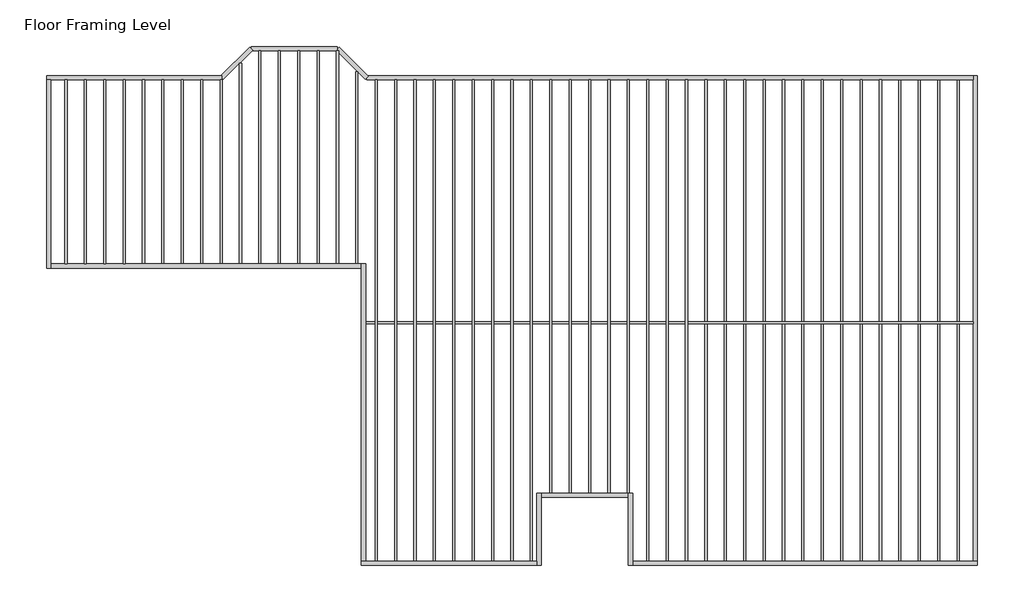
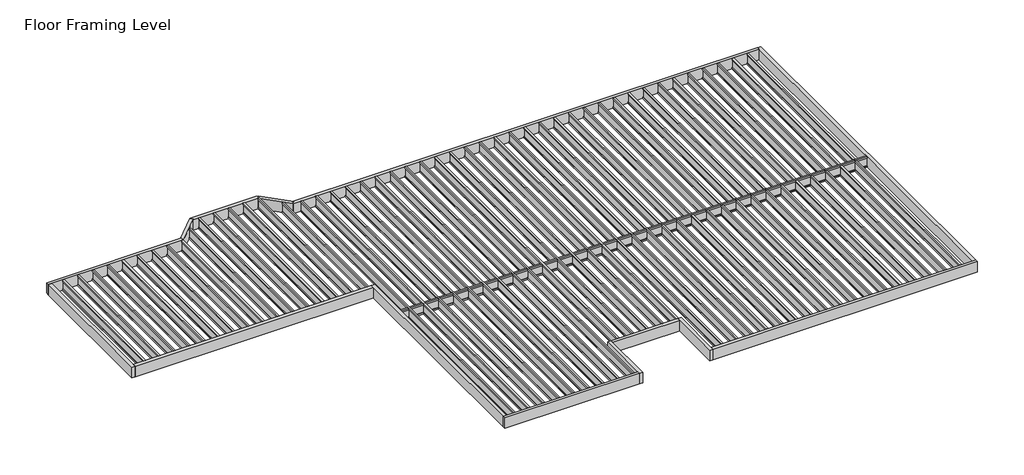
# One storey: 62 beams.
"""IFC4 building model written with IfcOpenShell, lengths in millimetres."""

import ifcopenshell
import ifcopenshell.guid

model = None  # the IFC model being written
_history = None  # IfcOwnerHistory: only IFC2X3 demands one
_inside = {}  # id of a spatial element -> (the spatial element, [elements in it])
_under = {}  # id of a project, library or spatial element -> (it, [spatial elements below it])
_declared = {}  # id of a project -> (the project, [libraries it declares])
_typed = {}  # id of a type object -> (the type object, [elements of that type])
_made_of = {}  # id of a material, layer set ... -> (it, [elements and type objects made of it])


def new_model(schema):
    """Start an empty IFC model of exactly this schema.

    Asked for "IFC4X3", IfcOpenShell would pick the latest addendum, in which some entities
    have other attributes; the version numbers below select the first issue.
    IFC2X3 requires an IfcOwnerHistory on every rooted entity: one is made here for all.
    """
    global model, _history
    if schema == "IFC4X3":
        model = ifcopenshell.file(schema_version=(4, 3, 0, 0))
    else:
        model = ifcopenshell.file(schema=schema)
    _inside.clear()
    _under.clear()
    _declared.clear()
    _typed.clear()
    _made_of.clear()
    _history = None
    if model.schema == "IFC2X3":
        org = make("IfcOrganization", Name="unknown")
        user = make(
            "IfcPersonAndOrganization",
            ThePerson=make("IfcPerson", FamilyName="unknown"),
            TheOrganization=org,
        )
        app = make(
            "IfcApplication",
            ApplicationDeveloper=org,
            Version="unknown",
            ApplicationFullName="unknown",
            ApplicationIdentifier="unknown",
        )
        _history = make(
            "IfcOwnerHistory",
            OwningUser=user,
            OwningApplication=app,
            ChangeAction="ADDED",
            CreationDate=0,
        )
    return model


def make(cls, **values):
    """One entity of the class cls with the attributes given. An attribute that is None is left unset."""
    return model.create_entity(
        cls, **{name: value for name, value in values.items() if value is not None}
    )


def rooted(cls, **values):
    """An entity with a GlobalId (a new one), such as an element, a storey or a relation."""
    return make(cls, GlobalId=ifcopenshell.guid.new(), OwnerHistory=_history, **values)


def si_unit(unit_type, name, prefix=None):
    """IfcSIUnit, for example si_unit("LENGTHUNIT", "METRE", prefix="MILLI")."""
    return make("IfcSIUnit", UnitType=unit_type, Prefix=prefix, Name=name)


def assignment(units):
    """IfcUnitAssignment: the units of a project."""
    return None if units is None else make("IfcUnitAssignment", Units=units)


def point(xyz):
    """IfcCartesianPoint."""
    return None if xyz is None else make("IfcCartesianPoint", Coordinates=xyz)


def direction(xyz):
    """IfcDirection."""
    return None if xyz is None else make("IfcDirection", DirectionRatios=xyz)


def frame(location, z_axis=None, x_axis=None):
    """IfcAxis2Placement3D, a coordinate frame: its origin and axes. An axis left out is left unset."""
    return make(
        "IfcAxis2Placement3D",
        Location=point(location),
        Axis=direction(z_axis),
        RefDirection=direction(x_axis),
    )


def origin():
    """The frame at (0, 0, 0) with its axes left unset."""
    return frame((0.0, 0.0, 0.0))


def place(relative_to, where):
    """IfcLocalPlacement: puts the frame where relative to a parent placement (None: the world)."""
    return make(
        "IfcLocalPlacement", PlacementRelTo=relative_to, RelativePlacement=where
    )


def context(
    kind, dimensions, precision=None, world=None, true_north=None, identifier=None
):
    """IfcGeometricRepresentationContext, for example the 3D "Model" context."""
    return make(
        "IfcGeometricRepresentationContext",
        ContextIdentifier=identifier,
        ContextType=kind,
        CoordinateSpaceDimension=dimensions,
        Precision=precision,
        WorldCoordinateSystem=world,
        TrueNorth=true_north,
    )


def project(units=None, contexts=None):
    """IfcProject with its units and contexts."""
    return rooted(
        "IfcProject",
        Name="project",
        RepresentationContexts=contexts,
        UnitsInContext=assignment(units),
    )


def spatial(cls, under=None, at=None, **own):
    """A site, building, storey or space (cls), placed at a placement, below another one or the project."""
    s = rooted(cls, ObjectPlacement=at, **own)
    if under is not None:
        _under.setdefault(under.id(), (under, []))[1].append(s)
    return s


def polyline(points):
    """IfcPolyline through the points."""
    return make("IfcPolyline", Points=[point(p) for p in points])


def outline(outer, holes=None, kind="AREA"):
    """IfcArbitraryClosedProfileDef: a profile drawn as a closed curve; with holes, ...WithVoids."""
    if holes is None:
        return make("IfcArbitraryClosedProfileDef", ProfileType=kind, OuterCurve=outer)
    return make(
        "IfcArbitraryProfileDefWithVoids",
        ProfileType=kind,
        OuterCurve=outer,
        InnerCurves=holes,
    )


def extrude(swept, where, along, depth):
    """IfcExtrudedAreaSolid: the profile swept, set in the frame where, extruded along a direction by depth."""
    return make(
        "IfcExtrudedAreaSolid",
        SweptArea=swept,
        Position=where,
        ExtrudedDirection=direction(along),
        Depth=depth,
    )


def shape(context_of_items, identifier, shape_type, items):
    """IfcShapeRepresentation: the items that make up one representation, for example the "Body"."""
    return make(
        "IfcShapeRepresentation",
        ContextOfItems=context_of_items,
        RepresentationIdentifier=identifier,
        RepresentationType=shape_type,
        Items=items,
    )


def source(mapping_origin, context_of_items, identifier, shape_type, items):
    """IfcRepresentationMap: a shape defined once, which mapped items show again and again."""
    return make(
        "IfcRepresentationMap",
        MappingOrigin=mapping_origin,
        MappedRepresentation=shape(context_of_items, identifier, shape_type, items),
    )


def transform(
    local_origin,
    x_axis=None,
    y_axis=None,
    z_axis=None,
    scale=None,
    scale2=None,
    scale3=None,
    uniform=True,
):
    """IfcCartesianTransformationOperator3D, or its non-uniform kind. x_axis, y_axis, z_axis: its Axis1, 2, 3."""
    if uniform:
        return make(
            "IfcCartesianTransformationOperator3D",
            Axis1=direction(x_axis),
            Axis2=direction(y_axis),
            LocalOrigin=point(local_origin),
            Scale=scale,
            Axis3=direction(z_axis),
        )
    return make(
        "IfcCartesianTransformationOperator3DnonUniform",
        Axis1=direction(x_axis),
        Axis2=direction(y_axis),
        LocalOrigin=point(local_origin),
        Scale=scale,
        Axis3=direction(z_axis),
        Scale2=scale2,
        Scale3=scale3,
    )


def mapped(mapping_source, mapping_target):
    """IfcMappedItem: shows the shape of a source again, moved by a transform."""
    return make(
        "IfcMappedItem", MappingSource=mapping_source, MappingTarget=mapping_target
    )


def made_of(thing, what):
    """Note that an element or type object is made of a material, layer set ...; save() writes the relation."""
    if what is not None:
        _made_of.setdefault(what.id(), (what, []))[1].append(thing)
    return thing


def element(
    cls,
    number,
    at=None,
    inside=None,
    cuts=None,
    type_object=None,
    material=None,
    context=None,
    identifier="Body",
    shape_type=None,
    held_by="IfcProductDefinitionShape",
    body=None,
    shapes=None,
    **own,
):
    """One element of the class cls, such as IfcWall. Its Tag is "e" and its number.

    at: its placement. inside: the storey or other place that contains it. cuts: it is an
    opening in that element (IfcRelVoidsElement). A single representation is given by context,
    identifier, shape_type and body (its items); several are given by shapes. held_by: the class
    of the entity that holds the representations. save() writes the other relations.
    """
    e = rooted(cls, Tag="e%d" % number, ObjectPlacement=at, **own)
    if body is not None:
        shapes = [shape(context, identifier, shape_type, body)]
    if shapes is not None:
        e.Representation = make(held_by, Representations=shapes)
    if inside is not None:
        _inside.setdefault(inside.id(), (inside, []))[1].append(e)
    if cuts is not None:
        rooted(
            "IfcRelVoidsElement", RelatingBuildingElement=cuts, RelatedOpeningElement=e
        )
    if type_object is not None:
        _typed.setdefault(type_object.id(), (type_object, []))[1].append(e)
    return made_of(e, material)


def aggregate(whole, parts):
    """IfcRelAggregates: a whole, such as a stair, and the parts it consists of."""
    return rooted("IfcRelAggregates", RelatingObject=whole, RelatedObjects=parts)


def save(model, path):
    """Write the relations noted so far, then the file.

    IfcRelAggregates (storeys below a building ...), IfcRelContainedInSpatialStructure (elements
    in a storey), IfcRelDefinesByType, IfcRelAssociatesMaterial and IfcRelDeclares: one each for
    every whole, place, type object, material and project.
    """
    for whole, parts in _under.values():
        aggregate(whole, parts)
    for where, things in _inside.values():
        rooted(
            "IfcRelContainedInSpatialStructure",
            RelatedElements=things,
            RelatingStructure=where,
        )
    for kind, things in _typed.values():
        rooted("IfcRelDefinesByType", RelatedObjects=things, RelatingType=kind)
    for what, things in _made_of.values():
        rooted("IfcRelAssociatesMaterial", RelatedObjects=things, RelatingMaterial=what)
    for by, libraries in _declared.values():
        rooted("IfcRelDeclares", RelatingContext=by, RelatedDefinitions=libraries)
    model.write(path)


def beam_585373de(model_context):
    return source(origin(), model_context, "Body", "SweptSolid", [
        extrude(outline(polyline([(755.65, 44.45), (755.65, -44.45), (-755.65, -44.45), (-755.65, 44.45), (755.65, 44.45)])), frame((0.0, 0.0, -150.8125), z_axis=(0.0, 0.0, 1.0), x_axis=(1.0, 0.0, 0.0)), (0.0, 0.0, 1.0), 301.625),
    ])


def beam_ce0f0212(model_context):
    return source(origin(), model_context, "Body", "SweptSolid", [
        extrude(outline(polyline([(5041.9, 44.45), (5041.9, -44.45), (-5130.8, -44.45), (-5130.8, 44.45), (5041.9, 44.45)])), frame((0.0, 0.0, -150.8125), z_axis=(0.0, 0.0, 1.0), x_axis=(1.0, 0.0, 0.0)), (0.0, 0.0, 1.0), 301.625),
    ])


def beam_45e17afb(model_context):
    return source(origin(), model_context, "Body", "SweptSolid", [
        extrude(outline(polyline([(3568.7, 44.45), (3568.7, -44.45), (-3657.6, -44.45), (-3657.6, 44.45), (3568.7, 44.45)])), frame((0.0, 0.0, -150.8125), z_axis=(0.0, 0.0, 1.0), x_axis=(1.0, 0.0, 0.0)), (0.0, 0.0, 1.0), 301.625),
    ])


def beam_b5369756(model_context):
    return source(origin(), model_context, "Body", "SweptSolid", [
        extrude(outline(polyline([(914.4, 44.45), (914.4, -44.45), (-914.4, -44.45), (-914.4, 44.45), (914.4, 44.45)])), frame((0.0, 0.0, -150.8125), z_axis=(0.0, 0.0, 1.0), x_axis=(1.0, 0.0, 0.0)), (0.0, 0.0, 1.0), 301.625),
    ])


def beam_28985cd7(model_context):
    return source(origin(), model_context, "Body", "SweptSolid", [
        extrude(outline(polyline([(1882.775, 44.45), (1882.775, -44.45), (-1793.875, -44.45), (-1793.875, 44.45), (1882.775, 44.45)])), frame((0.0, 0.0, -150.8125), z_axis=(0.0, 0.0, 1.0), x_axis=(1.0, 0.0, 0.0)), (0.0, 0.0, 1.0), 301.625),
    ])


def beam_51e41891(model_context):
    return source(origin(), model_context, "Body", "SweptSolid", [
        extrude(outline(polyline([(3159.125, 44.45), (3159.125, -44.45), (-3070.225, -44.45), (-3070.225, 44.45), (3159.125, 44.45)])), frame((0.0, 0.0, -150.8125), z_axis=(0.0, 0.0, 1.0), x_axis=(1.0, 0.0, 0.0)), (0.0, 0.0, 1.0), 301.625),
    ])


def beam_440427b1(model_context):
    return source(origin(), model_context, "Body", "SweptSolid", [
        extrude(outline(polyline([(3254.375, 44.45), (3254.375, -44.45), (-3254.375, -44.45), (-3254.375, 44.45), (3254.375, 44.45)])), frame((0.0, 0.0, -150.8125), z_axis=(0.0, 0.0, 1.0), x_axis=(1.0, 0.0, 0.0)), (0.0, 0.0, 1.0), 301.625),
    ])


def beam_dcf2d3fa(model_context):
    return source(origin(), model_context, "Body", "SweptSolid", [
        extrude(outline(polyline([(1927.225, 44.45), (1927.225, -44.45), (-2016.125, -44.45), (-2016.125, 44.45), (1927.225, 44.45)])), frame((0.0, 0.0, -150.8125), z_axis=(0.0, 0.0, 1.0), x_axis=(1.0, 0.0, 0.0)), (0.0, 0.0, 1.0), 301.625),
    ])


def beam_d6a2cfd4(model_context):
    return source(origin(), model_context, "Body", "SweptSolid", [
        extrude(outline(polyline([(431.0522938, 44.45), (431.0522938, -44.45), (-431.0522938, -44.45), (-431.0522938, 44.45), (431.0522938, 44.45)])), frame((0.0, 0.0, -150.8125), z_axis=(0.0, 0.0, 1.0), x_axis=(1.0, 0.0, 0.0)), (0.0, 0.0, 1.0), 301.625),
    ])


def beam_9835caef(model_context):
    return source(origin(), model_context, "Body", "SweptSolid", [
        extrude(outline(polyline([(1815.7808964, 44.45), (1815.7808964, -44.45), (-1860.2308964, -44.45), (-1860.2308964, 44.45), (1815.7808964, 44.45)])), frame((0.0, 0.0, -150.8125), z_axis=(0.0, 0.0, 1.0), x_axis=(1.0, 0.0, 0.0)), (0.0, 0.0, 1.0), 301.625),
    ])


def beam_6192414b(model_context):
    return source(origin(), model_context, "Body", "SweptSolid", [
        extrude(outline(polyline([(903.8789755, 44.45), (903.8789755, -44.45), (-906.5092316, -44.45), (-906.5092316, 44.45), (903.8789755, 44.45)])), frame((0.0, 0.0, -150.8125), z_axis=(0.0, 0.0, 1.0), x_axis=(1.0, 0.0, 0.0)), (0.0, 0.0, 1.0), 301.625),
    ])


def beam_06e53553(model_context):
    return source(origin(), model_context, "Body", "SweptSolid", [
        extrude(outline(polyline([(6332.8098719, 44.45), (6332.8098719, -44.45), (-6377.2598719, -44.45), (-6377.2598719, 44.45), (6332.8098719, 44.45)])), frame((0.0, 0.0, -150.8125), z_axis=(0.0, 0.0, 1.0), x_axis=(1.0, 0.0, 0.0)), (0.0, 0.0, 1.0), 301.625),
    ])


def plywood_web_joist_bldg_6241_1_3_4x11_7_8_b749f0c8(model_context):
    return source(origin(), model_context, "Body", "SweptSolid", [
        extrude(outline(polyline([(-22.225, 150.8125), (22.225, 150.8125), (22.225, 112.7125), (4.7625, 112.7125), (4.7625, 119.0625), (-4.7625, 119.0625), (-4.7625, 112.7125), (-22.225, 112.7125), (-22.225, 150.8125)])), frame((-5041.9, 0.0, 0.0), z_axis=(1.0, 0.0, 0.0), x_axis=(0.0, 1.0, 0.0)), (0.0, 0.0, 1.0), 10083.8),
        extrude(outline(polyline([(22.225, -112.7125), (22.225, -150.8125), (-22.225, -150.8125), (-22.225, -112.7125), (-4.7625, -112.7125), (-4.7625, -118.3285374), (4.7625, -118.3285374), (4.7625, -112.7125), (22.225, -112.7125)])), frame((-5041.9, 0.0, 0.0), z_axis=(1.0, 0.0, 0.0), x_axis=(0.0, 1.0, 0.0)), (0.0, 0.0, 1.0), 10083.8),
        extrude(outline(polyline([(5041.9, 4.7625), (5041.9, -4.7625), (-5041.9, -4.7625), (-5041.9, 4.7625), (5041.9, 4.7625)])), frame((0.0, 0.0, -118.3285374), z_axis=(0.0, 0.0, 1.0), x_axis=(1.0, 0.0, 0.0)), (0.0, 0.0, 1.0), 237.3910374),
    ])


def plywood_web_joist_bldg_6241_1_3_4x11_7_8_a6b37d20(model_context):
    return source(origin(), model_context, "Body", "SweptSolid", [
        extrude(outline(polyline([(-22.225, 150.8125), (22.225, 150.8125), (22.225, 112.7125), (4.7625, 112.7125), (4.7625, 119.0625), (-4.7625, 119.0625), (-4.7625, 112.7125), (-22.225, 112.7125), (-22.225, 150.8125)])), frame((-4330.7, 0.0, 0.0), z_axis=(1.0, 0.0, 0.0), x_axis=(0.0, 1.0, 0.0)), (0.0, 0.0, 1.0), 8661.4),
        extrude(outline(polyline([(22.225, -112.7125), (22.225, -150.8125), (-22.225, -150.8125), (-22.225, -112.7125), (-4.7625, -112.7125), (-4.7625, -118.3285374), (4.7625, -118.3285374), (4.7625, -112.7125), (22.225, -112.7125)])), frame((-4330.7, 0.0, 0.0), z_axis=(1.0, 0.0, 0.0), x_axis=(0.0, 1.0, 0.0)), (0.0, 0.0, 1.0), 8661.4),
        extrude(outline(polyline([(4330.7, 4.7625), (4330.7, -4.7625), (-4330.7, -4.7625), (-4330.7, 4.7625), (4330.7, 4.7625)])), frame((0.0, 0.0, -118.3285374), z_axis=(0.0, 0.0, 1.0), x_axis=(1.0, 0.0, 0.0)), (0.0, 0.0, 1.0), 237.3910374),
    ])


def plywood_web_joist_bldg_6241_1_3_4x11_7_8_9cf04d55(model_context):
    return source(origin(), model_context, "Body", "SweptSolid", [
        extrude(outline(polyline([(-22.225, 150.8125), (22.225, 150.8125), (22.225, 112.7125), (4.7625, 112.7125), (4.7625, 119.0625), (-4.7625, 119.0625), (-4.7625, 112.7125), (-22.225, 112.7125), (-22.225, 150.8125)])), frame((-1927.225, 0.0, 0.0), z_axis=(1.0, 0.0, 0.0), x_axis=(0.0, 1.0, 0.0)), (0.0, 0.0, 1.0), 3854.45),
        extrude(outline(polyline([(22.225, -112.7125), (22.225, -150.8125), (-22.225, -150.8125), (-22.225, -112.7125), (-4.7625, -112.7125), (-4.7625, -118.3285374), (4.7625, -118.3285374), (4.7625, -112.7125), (22.225, -112.7125)])), frame((-1927.225, 0.0, 0.0), z_axis=(1.0, 0.0, 0.0), x_axis=(0.0, 1.0, 0.0)), (0.0, 0.0, 1.0), 3854.45),
        extrude(outline(polyline([(1927.225, 4.7625), (1927.225, -4.7625), (-1927.225, -4.7625), (-1927.225, 4.7625), (1927.225, 4.7625)])), frame((0.0, 0.0, -118.3285374), z_axis=(0.0, 0.0, 1.0), x_axis=(1.0, 0.0, 0.0)), (0.0, 0.0, 1.0), 237.3910374),
    ])


def plywood_web_joist_bldg_6241_1_3_4x11_7_8_881987cb(model_context):
    return source(origin(), model_context, "Body", "SweptSolid", [
        extrude(outline(polyline([(-22.225, 150.8125), (22.225, 150.8125), (22.225, 112.7125), (4.7625, 112.7125), (4.7625, 119.0625), (-4.7625, 119.0625), (-4.7625, 112.7125), (-22.225, 112.7125), (-22.225, 150.8125)])), frame((-2121.2191036, 0.0, 0.0), z_axis=(1.0, 0.0, 0.0), x_axis=(0.0, 1.0, 0.0)), (0.0, 0.0, 1.0), 4201.8014143),
        extrude(outline(polyline([(22.225, -112.7125), (22.225, -150.8125), (-22.225, -150.8125), (-22.225, -112.7125), (-4.7625, -112.7125), (-4.7625, -118.3285374), (4.7625, -118.3285374), (4.7625, -112.7125), (22.225, -112.7125)])), frame((-2121.2191036, 0.0, 0.0), z_axis=(1.0, 0.0, 0.0), x_axis=(0.0, 1.0, 0.0)), (0.0, 0.0, 1.0), 4201.8014143),
        extrude(outline(polyline([(2080.5823107, 4.7625), (2080.5823107, -4.7625), (-2121.2191036, -4.7625), (-2121.2191036, 4.7625), (2080.5823107, 4.7625)])), frame((0.0, 0.0, -118.3285374), z_axis=(0.0, 0.0, 1.0), x_axis=(1.0, 0.0, 0.0)), (0.0, 0.0, 1.0), 237.3910374),
    ])


def plywood_web_joist_bldg_6241_1_3_4x11_7_8_a42695ab(model_context):
    return source(origin(), model_context, "Body", "SweptSolid", [
        extrude(outline(polyline([(-22.225, 150.8125), (22.225, 150.8125), (22.225, 112.7125), (4.7625, 112.7125), (4.7625, 119.0625), (-4.7625, 119.0625), (-4.7625, 112.7125), (-22.225, 112.7125), (-22.225, 150.8125)])), frame((-2232.025, 0.0, 0.0), z_axis=(1.0, 0.0, 0.0), x_axis=(0.0, 1.0, 0.0)), (0.0, 0.0, 1.0), 4464.05),
        extrude(outline(polyline([(22.225, -112.7125), (22.225, -150.8125), (-22.225, -150.8125), (-22.225, -112.7125), (-4.7625, -112.7125), (-4.7625, -118.3285374), (4.7625, -118.3285374), (4.7625, -112.7125), (22.225, -112.7125)])), frame((-2232.025, 0.0, 0.0), z_axis=(1.0, 0.0, 0.0), x_axis=(0.0, 1.0, 0.0)), (0.0, 0.0, 1.0), 4464.05),
        extrude(outline(polyline([(2232.025, 4.7625), (2232.025, -4.7625), (-2232.025, -4.7625), (-2232.025, 4.7625), (2232.025, 4.7625)])), frame((0.0, 0.0, -118.3285374), z_axis=(0.0, 0.0, 1.0), x_axis=(1.0, 0.0, 0.0)), (0.0, 0.0, 1.0), 237.3910374),
    ])


def plywood_web_joist_bldg_6241_1_3_4x11_7_8_0dc58311(model_context):
    return source(origin(), model_context, "Body", "SweptSolid", [
        extrude(outline(polyline([(-22.225, 150.8125), (22.225, 150.8125), (22.225, 112.7125), (4.7625, 112.7125), (4.7625, 119.0625), (-4.7625, 119.0625), (-4.7625, 112.7125), (-22.225, 112.7125), (-22.225, 150.8125)])), frame((-2030.1401281, 0.0, 0.0), z_axis=(1.0, 0.0, 0.0), x_axis=(0.0, 1.0, 0.0)), (0.0, 0.0, 1.0), 4019.6434633),
        extrude(outline(polyline([(22.225, -112.7125), (22.225, -150.8125), (-22.225, -150.8125), (-22.225, -112.7125), (-4.7625, -112.7125), (-4.7625, -118.3285374), (4.7625, -118.3285374), (4.7625, -112.7125), (22.225, -112.7125)])), frame((-2030.1401281, 0.0, 0.0), z_axis=(1.0, 0.0, 0.0), x_axis=(0.0, 1.0, 0.0)), (0.0, 0.0, 1.0), 4019.6434633),
        extrude(outline(polyline([(1989.5033352, 4.7625), (1989.5033352, -4.7625), (-2030.1401281, -4.7625), (-2030.1401281, 4.7625), (1989.5033352, 4.7625)])), frame((0.0, 0.0, -118.3285374), z_axis=(0.0, 0.0, 1.0), x_axis=(1.0, 0.0, 0.0)), (0.0, 0.0, 1.0), 237.3910374),
    ])


def plywood_web_joist_bldg_6241_1_3_4x11_7_8_0dbcbf17(model_context):
    return source(origin(), model_context, "Body", "SweptSolid", [
        extrude(outline(polyline([(-22.225, 150.8125), (22.225, 150.8125), (22.225, 112.7125), (4.7625, 112.7125), (4.7625, 119.0625), (-4.7625, 119.0625), (-4.7625, 112.7125), (-22.225, 112.7125), (-22.225, 150.8125)])), frame((-6365.875, 0.0, 0.0), z_axis=(1.0, 0.0, 0.0), x_axis=(0.0, 1.0, 0.0)), (0.0, 0.0, 1.0), 12731.75),
        extrude(outline(polyline([(22.225, -112.7125), (22.225, -150.8125), (-22.225, -150.8125), (-22.225, -112.7125), (-4.7625, -112.7125), (-4.7625, -118.3285374), (4.7625, -118.3285374), (4.7625, -112.7125), (22.225, -112.7125)])), frame((-6365.875, 0.0, 0.0), z_axis=(1.0, 0.0, 0.0), x_axis=(0.0, 1.0, 0.0)), (0.0, 0.0, 1.0), 12731.75),
        extrude(outline(polyline([(6365.875, 4.7625), (6365.875, -4.7625), (-6365.875, -4.7625), (-6365.875, 4.7625), (6365.875, 4.7625)])), frame((0.0, 0.0, -118.3285374), z_axis=(0.0, 0.0, 1.0), x_axis=(1.0, 0.0, 0.0)), (0.0, 0.0, 1.0), 237.3910374),
    ])


model = new_model("IFC4")

# Units and contexts
model_context = context("Model", 3, world=origin())
ifc_project = project(units=[si_unit("LENGTHUNIT", "METRE", prefix="MILLI")], contexts=[model_context])

# Site, building, storey
site = spatial("IfcSite", under=ifc_project)
building = spatial("IfcBuilding", under=site)
storey = spatial("IfcBuildingStorey", under=building, Name="Floor Framing Level", Elevation=-18.25625)

# Beams
placement = place(None, origin())
beam_shape = beam_585373de(model_context)
element("IfcBeam", 1, ObjectType="Dimension Lumber : BLDG 6241 Rim Board 11-7/8\"", at=placement, inside=storey, context=model_context, shape_type="MappedRepresentation", body=[
    mapped(beam_shape, transform((-5564.764829, -4298.2215886, -169.06875), x_axis=(0.0, 1.0, 0.0), y_axis=(-1.0, 0.0, 0.0), z_axis=(0.0, 0.0, 1.0))),
])
element("IfcBeam", 2, ObjectType="Dimension Lumber : BLDG 6241 Rim Board 11-7/8\"", at=placement, inside=storey, context=model_context, shape_type="MappedRepresentation", body=[
    mapped(beam_shape, transform((-7482.464829, -4298.2215886, -169.06875), x_axis=(0.0, -1.0, 0.0), y_axis=(1.0, 0.0, 0.0), z_axis=(0.0, 0.0, 1.0))),
])
beam_2_shape = beam_ce0f0212(model_context)
element("IfcBeam", 3, ObjectType="Dimension Lumber : BLDG 6241 Rim Board 11-7/8\"", at=placement, inside=storey, context=model_context, shape_type="MappedRepresentation", body=[
    mapped(beam_2_shape, transform((1661.535171, 76.9284114, -169.06875), x_axis=(0.0, -1.0, 0.0), y_axis=(1.0, 0.0, 0.0), z_axis=(0.0, 0.0, 1.0))),
])
beam_3_shape = beam_45e17afb(model_context)
element("IfcBeam", 4, ObjectType="Dimension Lumber : BLDG 6241 Rim Board 11-7/8\"", at=placement, inside=storey, context=model_context, shape_type="MappedRepresentation", body=[
    mapped(beam_3_shape, transform((-1951.614829, -5009.4215886, -169.06875), x_axis=(-1.0, 0.0, 0.0), y_axis=(0.0, -1.0, 0.0), z_axis=(0.0, 0.0, 1.0))),
])
beam_4_shape = beam_b5369756(model_context)
element("IfcBeam", 5, ObjectType="Dimension Lumber : BLDG 6241 Rim Board 11-7/8\"", at=placement, inside=storey, context=model_context, shape_type="MappedRepresentation", body=[
    mapped(beam_4_shape, transform((-6523.614829, -3587.0215886, -169.06875), x_axis=(-1.0, 0.0, 0.0), y_axis=(0.0, -1.0, 0.0), z_axis=(0.0, 0.0, 1.0))),
])
beam_5_shape = beam_28985cd7(model_context)
element("IfcBeam", 6, ObjectType="Dimension Lumber : BLDG 6241 Rim Board 11-7/8\"", at=placement, inside=storey, context=model_context, shape_type="MappedRepresentation", body=[
    mapped(beam_5_shape, transform((-9320.789829, -5009.4215886, -169.06875), x_axis=(-1.0, 0.0, 0.0), y_axis=(0.0, -1.0, 0.0), z_axis=(0.0, 0.0, 1.0))),
])
beam_6_shape = beam_51e41891(model_context)
element("IfcBeam", 7, ObjectType="Dimension Lumber : BLDG 6241 Rim Board 11-7/8\"", at=placement, inside=storey, context=model_context, shape_type="MappedRepresentation", body=[
    mapped(beam_6_shape, transform((-11159.114829, -1894.7465886, -169.06875), x_axis=(0.0, 1.0, 0.0), y_axis=(-1.0, 0.0, 0.0), z_axis=(0.0, 0.0, 1.0))),
])
beam_7_shape = beam_440427b1(model_context)
element("IfcBeam", 8, ObjectType="Dimension Lumber : BLDG 6241 Rim Board 11-7/8\"", at=placement, inside=storey, context=model_context, shape_type="MappedRepresentation", body=[
    mapped(beam_7_shape, transform((-14457.939829, 1219.9284114, -169.06875), x_axis=(-1.0, 0.0, 0.0), y_axis=(0.0, -1.0, 0.0), z_axis=(0.0, 0.0, 1.0))),
])
beam_8_shape = beam_dcf2d3fa(model_context)
element("IfcBeam", 9, ObjectType="Dimension Lumber : BLDG 6241 Rim Board 11-7/8\"", at=placement, inside=storey, context=model_context, shape_type="MappedRepresentation", body=[
    mapped(beam_8_shape, transform((-17756.764829, 3191.6034114, -169.06875), x_axis=(0.0, 1.0, 0.0), y_axis=(-1.0, 0.0, 0.0), z_axis=(0.0, 0.0, 1.0))),
])
beam_9_shape = beam_d6a2cfd4(model_context)
element("IfcBeam", 10, ObjectType="Dimension Lumber : BLDG 6241 Rim Board 11-7/8\"", at=placement, inside=storey, context=model_context, shape_type="MappedRepresentation", body=[
    mapped(beam_9_shape, transform((-13820.4030362, 5468.0784114, -169.06875), x_axis=(0.7071067811865488, 0.7071067811865464, 0.0), y_axis=(-0.7071067811865464, 0.7071067811865488, 0.0), z_axis=(0.0, 0.0, 1.0))),
])
element("IfcBeam", 11, ObjectType="Dimension Lumber : BLDG 6241 Rim Board 11-7/8\"", at=placement, inside=storey, context=model_context, shape_type="MappedRepresentation", body=[
    mapped(beam_9_shape, transform((-11397.7845729, 5468.0784114, -169.06875), x_axis=(0.7071067811865457, -0.7071067811865493, 0.0), y_axis=(0.7071067811865493, 0.7071067811865457, 0.0), z_axis=(0.0, 0.0, 1.0))),
])
beam_10_shape = beam_9835caef(model_context)
element("IfcBeam", 12, ObjectType="Dimension Lumber : BLDG 6241 Rim Board 11-7/8\"", at=placement, inside=storey, context=model_context, shape_type="MappedRepresentation", body=[
    mapped(beam_10_shape, transform((-15940.9839326, 5163.2784114, -169.06875), x_axis=(1.0, 0.0, 0.0), y_axis=(0.0, 1.0, 0.0), z_axis=(0.0, 0.0, 1.0))),
])
beam_11_shape = beam_6192414b(model_context)
element("IfcBeam", 13, ObjectType="Dimension Lumber : BLDG 6241 Rim Board 11-7/8\"", at=placement, inside=storey, context=model_context, shape_type="MappedRepresentation", body=[
    mapped(beam_11_shape, transform((-12609.0938046, 5772.8784114, -169.06875), x_axis=(1.0, 0.0, 0.0), y_axis=(0.0, 1.0, 0.0), z_axis=(0.0, 0.0, 1.0))),
])
beam_12_shape = beam_06e53553(model_context)
element("IfcBeam", 14, ObjectType="Dimension Lumber : BLDG 6241 Rim Board 11-7/8\"", at=placement, inside=storey, context=model_context, shape_type="MappedRepresentation", body=[
    mapped(beam_12_shape, transform((-4715.724701, 5163.2784114, -169.06875), x_axis=(1.0, 0.0, 0.0), y_axis=(0.0, 1.0, 0.0), z_axis=(0.0, 0.0, 1.0))),
])
plywood_web_joist_bldg_6241_1_3_4x11_7_8_shape = plywood_web_joist_bldg_6241_1_3_4x11_7_8_b749f0c8(model_context)
element("IfcBeam", 15, ObjectType="Plywood Web Joist : BLDG 6241 1 3/4x11 7/8", at=placement, inside=storey, context=model_context, shape_type="MappedRepresentation", body=[
    mapped(plywood_web_joist_bldg_6241_1_3_4x11_7_8_shape, transform((-10892.414829, 76.9284114, -169.06875), x_axis=(0.0, 1.0, 0.0), y_axis=(-1.0, 0.0, 0.0), z_axis=(0.0, 0.0, 1.0))),
])
element("IfcBeam", 16, ObjectType="Plywood Web Joist : BLDG 6241 1 3/4x11 7/8", at=placement, inside=storey, context=model_context, shape_type="MappedRepresentation", body=[
    mapped(plywood_web_joist_bldg_6241_1_3_4x11_7_8_shape, transform((-10486.014829, 76.9284114, -169.06875), x_axis=(0.0, 1.0, 0.0), y_axis=(-1.0, 0.0, 0.0), z_axis=(0.0, 0.0, 1.0))),
])
element("IfcBeam", 17, ObjectType="Plywood Web Joist : BLDG 6241 1 3/4x11 7/8", at=placement, inside=storey, context=model_context, shape_type="MappedRepresentation", body=[
    mapped(plywood_web_joist_bldg_6241_1_3_4x11_7_8_shape, transform((-10079.614829, 76.9284114, -169.06875), x_axis=(0.0, 1.0, 0.0), y_axis=(-1.0, 0.0, 0.0), z_axis=(0.0, 0.0, 1.0))),
])
element("IfcBeam", 18, ObjectType="Plywood Web Joist : BLDG 6241 1 3/4x11 7/8", at=placement, inside=storey, context=model_context, shape_type="MappedRepresentation", body=[
    mapped(plywood_web_joist_bldg_6241_1_3_4x11_7_8_shape, transform((-9673.214829, 76.9284114, -169.06875), x_axis=(0.0, 1.0, 0.0), y_axis=(-1.0, 0.0, 0.0), z_axis=(0.0, 0.0, 1.0))),
])
element("IfcBeam", 19, ObjectType="Plywood Web Joist : BLDG 6241 1 3/4x11 7/8", at=placement, inside=storey, context=model_context, shape_type="MappedRepresentation", body=[
    mapped(plywood_web_joist_bldg_6241_1_3_4x11_7_8_shape, transform((-9266.814829, 76.9284114, -169.06875), x_axis=(0.0, 1.0, 0.0), y_axis=(-1.0, 0.0, 0.0), z_axis=(0.0, 0.0, 1.0))),
])
element("IfcBeam", 20, ObjectType="Plywood Web Joist : BLDG 6241 1 3/4x11 7/8", at=placement, inside=storey, context=model_context, shape_type="MappedRepresentation", body=[
    mapped(plywood_web_joist_bldg_6241_1_3_4x11_7_8_shape, transform((-8860.414829, 76.9284114, -169.06875), x_axis=(0.0, 1.0, 0.0), y_axis=(-1.0, 0.0, 0.0), z_axis=(0.0, 0.0, 1.0))),
])
element("IfcBeam", 21, ObjectType="Plywood Web Joist : BLDG 6241 1 3/4x11 7/8", at=placement, inside=storey, context=model_context, shape_type="MappedRepresentation", body=[
    mapped(plywood_web_joist_bldg_6241_1_3_4x11_7_8_shape, transform((-8454.014829, 76.9284114, -169.06875), x_axis=(0.0, 1.0, 0.0), y_axis=(-1.0, 0.0, 0.0), z_axis=(0.0, 0.0, 1.0))),
])
element("IfcBeam", 22, ObjectType="Plywood Web Joist : BLDG 6241 1 3/4x11 7/8", at=placement, inside=storey, context=model_context, shape_type="MappedRepresentation", body=[
    mapped(plywood_web_joist_bldg_6241_1_3_4x11_7_8_shape, transform((-8047.614829, 76.9284114, -169.06875), x_axis=(0.0, 1.0, 0.0), y_axis=(-1.0, 0.0, 0.0), z_axis=(0.0, 0.0, 1.0))),
])
element("IfcBeam", 23, ObjectType="Plywood Web Joist : BLDG 6241 1 3/4x11 7/8", at=placement, inside=storey, context=model_context, shape_type="MappedRepresentation", body=[
    mapped(plywood_web_joist_bldg_6241_1_3_4x11_7_8_shape, transform((-7641.214829, 76.9284114, -169.06875), x_axis=(0.0, 1.0, 0.0), y_axis=(-1.0, 0.0, 0.0), z_axis=(0.0, 0.0, 1.0))),
])
element("IfcBeam", 24, ObjectType="Plywood Web Joist : BLDG 6241 1 3/4x11 7/8", at=placement, inside=storey, context=model_context, shape_type="MappedRepresentation", body=[
    mapped(plywood_web_joist_bldg_6241_1_3_4x11_7_8_shape, transform((-5202.814829, 76.9284114, -169.06875), x_axis=(0.0, 1.0, 0.0), y_axis=(-1.0, 0.0, 0.0), z_axis=(0.0, 0.0, 1.0))),
])
element("IfcBeam", 25, ObjectType="Plywood Web Joist : BLDG 6241 1 3/4x11 7/8", at=placement, inside=storey, context=model_context, shape_type="MappedRepresentation", body=[
    mapped(plywood_web_joist_bldg_6241_1_3_4x11_7_8_shape, transform((-4796.414829, 76.9284114, -169.06875), x_axis=(0.0, 1.0, 0.0), y_axis=(-1.0, 0.0, 0.0), z_axis=(0.0, 0.0, 1.0))),
])
element("IfcBeam", 26, ObjectType="Plywood Web Joist : BLDG 6241 1 3/4x11 7/8", at=placement, inside=storey, context=model_context, shape_type="MappedRepresentation", body=[
    mapped(plywood_web_joist_bldg_6241_1_3_4x11_7_8_shape, transform((-4390.014829, 76.9284114, -169.06875), x_axis=(0.0, 1.0, 0.0), y_axis=(-1.0, 0.0, 0.0), z_axis=(0.0, 0.0, 1.0))),
])
element("IfcBeam", 27, ObjectType="Plywood Web Joist : BLDG 6241 1 3/4x11 7/8", at=placement, inside=storey, context=model_context, shape_type="MappedRepresentation", body=[
    mapped(plywood_web_joist_bldg_6241_1_3_4x11_7_8_shape, transform((-3983.614829, 76.9284114, -169.06875), x_axis=(0.0, 1.0, 0.0), y_axis=(-1.0, 0.0, 0.0), z_axis=(0.0, 0.0, 1.0))),
])
element("IfcBeam", 28, ObjectType="Plywood Web Joist : BLDG 6241 1 3/4x11 7/8", at=placement, inside=storey, context=model_context, shape_type="MappedRepresentation", body=[
    mapped(plywood_web_joist_bldg_6241_1_3_4x11_7_8_shape, transform((-3577.214829, 76.9284114, -169.06875), x_axis=(0.0, 1.0, 0.0), y_axis=(-1.0, 0.0, 0.0), z_axis=(0.0, 0.0, 1.0))),
])
element("IfcBeam", 29, ObjectType="Plywood Web Joist : BLDG 6241 1 3/4x11 7/8", at=placement, inside=storey, context=model_context, shape_type="MappedRepresentation", body=[
    mapped(plywood_web_joist_bldg_6241_1_3_4x11_7_8_shape, transform((-3170.814829, 76.9284114, -169.06875), x_axis=(0.0, 1.0, 0.0), y_axis=(-1.0, 0.0, 0.0), z_axis=(0.0, 0.0, 1.0))),
])
element("IfcBeam", 30, ObjectType="Plywood Web Joist : BLDG 6241 1 3/4x11 7/8", at=placement, inside=storey, context=model_context, shape_type="MappedRepresentation", body=[
    mapped(plywood_web_joist_bldg_6241_1_3_4x11_7_8_shape, transform((-2764.414829, 76.9284114, -169.06875), x_axis=(0.0, 1.0, 0.0), y_axis=(-1.0, 0.0, 0.0), z_axis=(0.0, 0.0, 1.0))),
])
element("IfcBeam", 31, ObjectType="Plywood Web Joist : BLDG 6241 1 3/4x11 7/8", at=placement, inside=storey, context=model_context, shape_type="MappedRepresentation", body=[
    mapped(plywood_web_joist_bldg_6241_1_3_4x11_7_8_shape, transform((-2358.014829, 76.9284114, -169.06875), x_axis=(0.0, 1.0, 0.0), y_axis=(-1.0, 0.0, 0.0), z_axis=(0.0, 0.0, 1.0))),
])
element("IfcBeam", 32, ObjectType="Plywood Web Joist : BLDG 6241 1 3/4x11 7/8", at=placement, inside=storey, context=model_context, shape_type="MappedRepresentation", body=[
    mapped(plywood_web_joist_bldg_6241_1_3_4x11_7_8_shape, transform((-1951.614829, 76.9284114, -169.06875), x_axis=(0.0, 1.0, 0.0), y_axis=(-1.0, 0.0, 0.0), z_axis=(0.0, 0.0, 1.0))),
])
element("IfcBeam", 33, ObjectType="Plywood Web Joist : BLDG 6241 1 3/4x11 7/8", at=placement, inside=storey, context=model_context, shape_type="MappedRepresentation", body=[
    mapped(plywood_web_joist_bldg_6241_1_3_4x11_7_8_shape, transform((-1545.214829, 76.9284114, -169.06875), x_axis=(0.0, 1.0, 0.0), y_axis=(-1.0, 0.0, 0.0), z_axis=(0.0, 0.0, 1.0))),
])
element("IfcBeam", 34, ObjectType="Plywood Web Joist : BLDG 6241 1 3/4x11 7/8", at=placement, inside=storey, context=model_context, shape_type="MappedRepresentation", body=[
    mapped(plywood_web_joist_bldg_6241_1_3_4x11_7_8_shape, transform((-1138.814829, 76.9284114, -169.06875), x_axis=(0.0, 1.0, 0.0), y_axis=(-1.0, 0.0, 0.0), z_axis=(0.0, 0.0, 1.0))),
])
element("IfcBeam", 35, ObjectType="Plywood Web Joist : BLDG 6241 1 3/4x11 7/8", at=placement, inside=storey, context=model_context, shape_type="MappedRepresentation", body=[
    mapped(plywood_web_joist_bldg_6241_1_3_4x11_7_8_shape, transform((-732.414829, 76.9284114, -169.06875), x_axis=(0.0, 1.0, 0.0), y_axis=(-1.0, 0.0, 0.0), z_axis=(0.0, 0.0, 1.0))),
])
element("IfcBeam", 36, ObjectType="Plywood Web Joist : BLDG 6241 1 3/4x11 7/8", at=placement, inside=storey, context=model_context, shape_type="MappedRepresentation", body=[
    mapped(plywood_web_joist_bldg_6241_1_3_4x11_7_8_shape, transform((-326.014829, 76.9284114, -169.06875), x_axis=(0.0, 1.0, 0.0), y_axis=(-1.0, 0.0, 0.0), z_axis=(0.0, 0.0, 1.0))),
])
element("IfcBeam", 37, ObjectType="Plywood Web Joist : BLDG 6241 1 3/4x11 7/8", at=placement, inside=storey, context=model_context, shape_type="MappedRepresentation", body=[
    mapped(plywood_web_joist_bldg_6241_1_3_4x11_7_8_shape, transform((80.385171, 76.9284114, -169.06875), x_axis=(0.0, 1.0, 0.0), y_axis=(-1.0, 0.0, 0.0), z_axis=(0.0, 0.0, 1.0))),
])
element("IfcBeam", 38, ObjectType="Plywood Web Joist : BLDG 6241 1 3/4x11 7/8", at=placement, inside=storey, context=model_context, shape_type="MappedRepresentation", body=[
    mapped(plywood_web_joist_bldg_6241_1_3_4x11_7_8_shape, transform((486.785171, 76.9284114, -169.06875), x_axis=(0.0, 1.0, 0.0), y_axis=(-1.0, 0.0, 0.0), z_axis=(0.0, 0.0, 1.0))),
])
element("IfcBeam", 39, ObjectType="Plywood Web Joist : BLDG 6241 1 3/4x11 7/8", at=placement, inside=storey, context=model_context, shape_type="MappedRepresentation", body=[
    mapped(plywood_web_joist_bldg_6241_1_3_4x11_7_8_shape, transform((893.185171, 76.9284114, -169.06875), x_axis=(0.0, 1.0, 0.0), y_axis=(-1.0, 0.0, 0.0), z_axis=(0.0, 0.0, 1.0))),
])
element("IfcBeam", 40, ObjectType="Plywood Web Joist : BLDG 6241 1 3/4x11 7/8", at=placement, inside=storey, context=model_context, shape_type="MappedRepresentation", body=[
    mapped(plywood_web_joist_bldg_6241_1_3_4x11_7_8_shape, transform((1299.585171, 76.9284114, -169.06875), x_axis=(0.0, 1.0, 0.0), y_axis=(-1.0, 0.0, 0.0), z_axis=(0.0, 0.0, 1.0))),
])
plywood_web_joist_bldg_6241_1_3_4x11_7_8_2_shape = plywood_web_joist_bldg_6241_1_3_4x11_7_8_a6b37d20(model_context)
element("IfcBeam", 41, ObjectType="Plywood Web Joist : BLDG 6241 1 3/4x11 7/8", at=placement, inside=storey, context=model_context, shape_type="MappedRepresentation", body=[
    mapped(plywood_web_joist_bldg_6241_1_3_4x11_7_8_2_shape, transform((-7234.814829, 788.1284114, -169.06875), x_axis=(0.0, 1.0, 0.0), y_axis=(-1.0, 0.0, 0.0), z_axis=(0.0, 0.0, 1.0))),
])
element("IfcBeam", 42, ObjectType="Plywood Web Joist : BLDG 6241 1 3/4x11 7/8", at=placement, inside=storey, context=model_context, shape_type="MappedRepresentation", body=[
    mapped(plywood_web_joist_bldg_6241_1_3_4x11_7_8_2_shape, transform((-6828.414829, 788.1284114, -169.06875), x_axis=(0.0, 1.0, 0.0), y_axis=(-1.0, 0.0, 0.0), z_axis=(0.0, 0.0, 1.0))),
])
element("IfcBeam", 43, ObjectType="Plywood Web Joist : BLDG 6241 1 3/4x11 7/8", at=placement, inside=storey, context=model_context, shape_type="MappedRepresentation", body=[
    mapped(plywood_web_joist_bldg_6241_1_3_4x11_7_8_2_shape, transform((-6422.014829, 788.1284114, -169.06875), x_axis=(0.0, 1.0, 0.0), y_axis=(-1.0, 0.0, 0.0), z_axis=(0.0, 0.0, 1.0))),
])
element("IfcBeam", 44, ObjectType="Plywood Web Joist : BLDG 6241 1 3/4x11 7/8", at=placement, inside=storey, context=model_context, shape_type="MappedRepresentation", body=[
    mapped(plywood_web_joist_bldg_6241_1_3_4x11_7_8_2_shape, transform((-6015.614829, 788.1284114, -169.06875), x_axis=(0.0, 1.0, 0.0), y_axis=(-1.0, 0.0, 0.0), z_axis=(0.0, 0.0, 1.0))),
])
element("IfcBeam", 45, ObjectType="Plywood Web Joist : BLDG 6241 1 3/4x11 7/8", at=placement, inside=storey, context=model_context, shape_type="MappedRepresentation", body=[
    mapped(plywood_web_joist_bldg_6241_1_3_4x11_7_8_2_shape, transform((-5609.214829, 788.1284114, -169.06875), x_axis=(0.0, 1.0, 0.0), y_axis=(-1.0, 0.0, 0.0), z_axis=(0.0, 0.0, 1.0))),
])
plywood_web_joist_bldg_6241_1_3_4x11_7_8_3_shape = plywood_web_joist_bldg_6241_1_3_4x11_7_8_9cf04d55(model_context)
element("IfcBeam", 46, ObjectType="Plywood Web Joist : BLDG 6241 1 3/4x11 7/8", at=placement, inside=storey, context=model_context, shape_type="MappedRepresentation", body=[
    mapped(plywood_web_joist_bldg_6241_1_3_4x11_7_8_3_shape, transform((-17394.814829, 3191.6034114, -169.06875), x_axis=(0.0, 1.0, 0.0), y_axis=(-1.0, 0.0, 0.0), z_axis=(0.0, 0.0, 1.0))),
])
element("IfcBeam", 47, ObjectType="Plywood Web Joist : BLDG 6241 1 3/4x11 7/8", at=placement, inside=storey, context=model_context, shape_type="MappedRepresentation", body=[
    mapped(plywood_web_joist_bldg_6241_1_3_4x11_7_8_3_shape, transform((-16988.414829, 3191.6034114, -169.06875), x_axis=(0.0, 1.0, 0.0), y_axis=(-1.0, 0.0, 0.0), z_axis=(0.0, 0.0, 1.0))),
])
element("IfcBeam", 48, ObjectType="Plywood Web Joist : BLDG 6241 1 3/4x11 7/8", at=placement, inside=storey, context=model_context, shape_type="MappedRepresentation", body=[
    mapped(plywood_web_joist_bldg_6241_1_3_4x11_7_8_3_shape, transform((-16582.014829, 3191.6034114, -169.06875), x_axis=(0.0, 1.0, 0.0), y_axis=(-1.0, 0.0, 0.0), z_axis=(0.0, 0.0, 1.0))),
])
element("IfcBeam", 49, ObjectType="Plywood Web Joist : BLDG 6241 1 3/4x11 7/8", at=placement, inside=storey, context=model_context, shape_type="MappedRepresentation", body=[
    mapped(plywood_web_joist_bldg_6241_1_3_4x11_7_8_3_shape, transform((-16175.614829, 3191.6034114, -169.06875), x_axis=(0.0, 1.0, 0.0), y_axis=(-1.0, 0.0, 0.0), z_axis=(0.0, 0.0, 1.0))),
])
element("IfcBeam", 50, ObjectType="Plywood Web Joist : BLDG 6241 1 3/4x11 7/8", at=placement, inside=storey, context=model_context, shape_type="MappedRepresentation", body=[
    mapped(plywood_web_joist_bldg_6241_1_3_4x11_7_8_3_shape, transform((-15769.214829, 3191.6034114, -169.06875), x_axis=(0.0, 1.0, 0.0), y_axis=(-1.0, 0.0, 0.0), z_axis=(0.0, 0.0, 1.0))),
])
element("IfcBeam", 51, ObjectType="Plywood Web Joist : BLDG 6241 1 3/4x11 7/8", at=placement, inside=storey, context=model_context, shape_type="MappedRepresentation", body=[
    mapped(plywood_web_joist_bldg_6241_1_3_4x11_7_8_3_shape, transform((-15362.814829, 3191.6034114, -169.06875), x_axis=(0.0, 1.0, 0.0), y_axis=(-1.0, 0.0, 0.0), z_axis=(0.0, 0.0, 1.0))),
])
element("IfcBeam", 52, ObjectType="Plywood Web Joist : BLDG 6241 1 3/4x11 7/8", at=placement, inside=storey, context=model_context, shape_type="MappedRepresentation", body=[
    mapped(plywood_web_joist_bldg_6241_1_3_4x11_7_8_3_shape, transform((-14956.414829, 3191.6034114, -169.06875), x_axis=(0.0, 1.0, 0.0), y_axis=(-1.0, 0.0, 0.0), z_axis=(0.0, 0.0, 1.0))),
])
element("IfcBeam", 53, ObjectType="Plywood Web Joist : BLDG 6241 1 3/4x11 7/8", at=placement, inside=storey, context=model_context, shape_type="MappedRepresentation", body=[
    mapped(plywood_web_joist_bldg_6241_1_3_4x11_7_8_3_shape, transform((-14550.014829, 3191.6034114, -169.06875), x_axis=(0.0, 1.0, 0.0), y_axis=(-1.0, 0.0, 0.0), z_axis=(0.0, 0.0, 1.0))),
])
element("IfcBeam", 54, ObjectType="Plywood Web Joist : BLDG 6241 1 3/4x11 7/8", at=placement, inside=storey, context=model_context, shape_type="MappedRepresentation", body=[
    mapped(plywood_web_joist_bldg_6241_1_3_4x11_7_8_3_shape, transform((-14143.614829, 3191.6034114, -169.06875), x_axis=(0.0, 1.0, 0.0), y_axis=(-1.0, 0.0, 0.0), z_axis=(0.0, 0.0, 1.0))),
])
plywood_web_joist_bldg_6241_1_3_4x11_7_8_4_shape = plywood_web_joist_bldg_6241_1_3_4x11_7_8_881987cb(model_context)
element("IfcBeam", 55, ObjectType="Plywood Web Joist : BLDG 6241 1 3/4x11 7/8", at=placement, inside=storey, context=model_context, shape_type="MappedRepresentation", body=[
    mapped(plywood_web_joist_bldg_6241_1_3_4x11_7_8_4_shape, transform((-13737.214829, 3385.5975149, -169.06875), x_axis=(0.0, 1.0, 0.0), y_axis=(-1.0, 0.0, 0.0), z_axis=(0.0, 0.0, 1.0))),
])
plywood_web_joist_bldg_6241_1_3_4x11_7_8_5_shape = plywood_web_joist_bldg_6241_1_3_4x11_7_8_a42695ab(model_context)
element("IfcBeam", 56, ObjectType="Plywood Web Joist : BLDG 6241 1 3/4x11 7/8", at=placement, inside=storey, context=model_context, shape_type="MappedRepresentation", body=[
    mapped(plywood_web_joist_bldg_6241_1_3_4x11_7_8_5_shape, transform((-13330.814829, 3496.4034114, -169.06875), x_axis=(0.0, 1.0, 0.0), y_axis=(-1.0, 0.0, 0.0), z_axis=(0.0, 0.0, 1.0))),
])
element("IfcBeam", 57, ObjectType="Plywood Web Joist : BLDG 6241 1 3/4x11 7/8", at=placement, inside=storey, context=model_context, shape_type="MappedRepresentation", body=[
    mapped(plywood_web_joist_bldg_6241_1_3_4x11_7_8_5_shape, transform((-12924.414829, 3496.4034114, -169.06875), x_axis=(0.0, 1.0, 0.0), y_axis=(-1.0, 0.0, 0.0), z_axis=(0.0, 0.0, 1.0))),
])
element("IfcBeam", 58, ObjectType="Plywood Web Joist : BLDG 6241 1 3/4x11 7/8", at=placement, inside=storey, context=model_context, shape_type="MappedRepresentation", body=[
    mapped(plywood_web_joist_bldg_6241_1_3_4x11_7_8_5_shape, transform((-12518.014829, 3496.4034114, -169.06875), x_axis=(0.0, 1.0, 0.0), y_axis=(-1.0, 0.0, 0.0), z_axis=(0.0, 0.0, 1.0))),
])
element("IfcBeam", 59, ObjectType="Plywood Web Joist : BLDG 6241 1 3/4x11 7/8", at=placement, inside=storey, context=model_context, shape_type="MappedRepresentation", body=[
    mapped(plywood_web_joist_bldg_6241_1_3_4x11_7_8_5_shape, transform((-12111.614829, 3496.4034114, -169.06875), x_axis=(0.0, 1.0, 0.0), y_axis=(-1.0, 0.0, 0.0), z_axis=(0.0, 0.0, 1.0))),
])
element("IfcBeam", 60, ObjectType="Plywood Web Joist : BLDG 6241 1 3/4x11 7/8", at=placement, inside=storey, context=model_context, shape_type="MappedRepresentation", body=[
    mapped(plywood_web_joist_bldg_6241_1_3_4x11_7_8_5_shape, transform((-11705.214829, 3496.4034114, -169.06875), x_axis=(0.0, 1.0, 0.0), y_axis=(-1.0, 0.0, 0.0), z_axis=(0.0, 0.0, 1.0))),
])
plywood_web_joist_bldg_6241_1_3_4x11_7_8_6_shape = plywood_web_joist_bldg_6241_1_3_4x11_7_8_0dc58311(model_context)
element("IfcBeam", 61, ObjectType="Plywood Web Joist : BLDG 6241 1 3/4x11 7/8", at=placement, inside=storey, context=model_context, shape_type="MappedRepresentation", body=[
    mapped(plywood_web_joist_bldg_6241_1_3_4x11_7_8_6_shape, transform((-11298.814829, 3294.5185394, -169.06875), x_axis=(0.0, 1.0, 0.0), y_axis=(-1.0, 0.0, 0.0), z_axis=(0.0, 0.0, 1.0))),
])
plywood_web_joist_bldg_6241_1_3_4x11_7_8_7_shape = plywood_web_joist_bldg_6241_1_3_4x11_7_8_0dbcbf17(model_context)
element("IfcBeam", 62, ObjectType="Plywood Web Joist : BLDG 6241 1 3/4x11 7/8", at=placement, inside=storey, context=model_context, shape_type="MappedRepresentation", body=[
    mapped(plywood_web_joist_bldg_6241_1_3_4x11_7_8_7_shape, transform((-4748.789829, 26.1284114, -169.06875), x_axis=(-1.0, 0.0, 0.0), y_axis=(0.0, -1.0, 0.0), z_axis=(0.0, 0.0, 1.0))),
])

save(model, "model.ifc")

# Revit data of these elements
# Type "Dimension Lumber : BLDG 6241 Rim Board 11-7/8\""
#   Assembly Code = "B10"
#   A = 0.273472 SF
#   Length [instance default] = 5' - 0"
#   b = 0' - 3 1/2"
#   d = 0' - 11 7/8"
#   Structural Material [instance default] = Softwood, Lumber
# Type "Plywood Web Joist : BLDG 6241 1 3/4x11 7/8"
#   Assembly Code = "B10"
#   Length [instance default] = 5' - 0"
#   b = 0' - 1 3/4"
#   d = 0' - 11 7/8"
#   Structural Material [instance default] = Softwood, Lumber
# Elements 1, 2, 3, 4, 5, 6, 7, 8, 9, 10, 11, 12, 13, 14 (IfcBeam, "Dimension Lumber : BLDG 6241 Rim Board 11-7/8\"")
#   Comments = ""
#   Structural Material = Softwood, Lumber
#   Phase Created = New Construction
#   Materials on its faces: "Softwood, Lumber"
# Elements 15, 16, 17, 18, 19, 20, 21, 22, 23, 24, 25, 26, 27, 28, 29, 30, 31, 32, 33, 34, 35, 36, 37, 38, 39, 40, 41, 42, 43, 44, 45, 46, 47, 48, 49, 50, 51, 52, 53, 54, 55, 56, 57, 58, 59, 60, 61 (IfcBeam, "Plywood Web Joist : BLDG 6241 1 3/4x11 7/8")
#   Structural Material = Softwood, Lumber
#   Phase Created = New Construction
#   Materials on its faces: "Softwood, Lumber"
# Element 62 (IfcBeam, "Plywood Web Joist : BLDG 6241 1 3/4x11 7/8")
#   Comments = ""
#   Structural Material = Softwood, Lumber
#   Phase Created = New Construction
#   Materials on its faces: "Softwood, Lumber"
# Materials
#   "Softwood, Lumber": class "Wood", colour RGB 223 192 134, transparency 0, Description = "Pinus Echinata", Cost = 0
